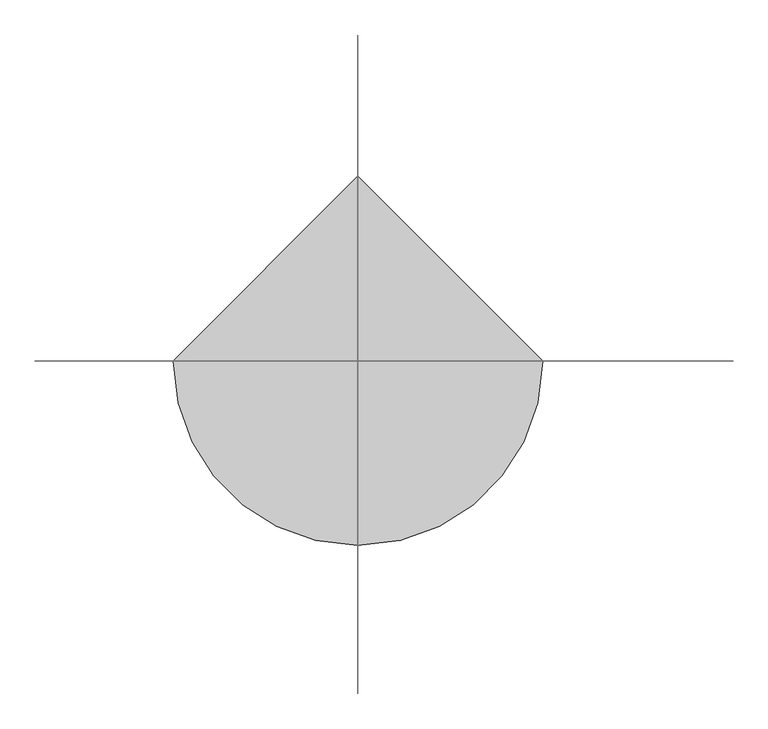
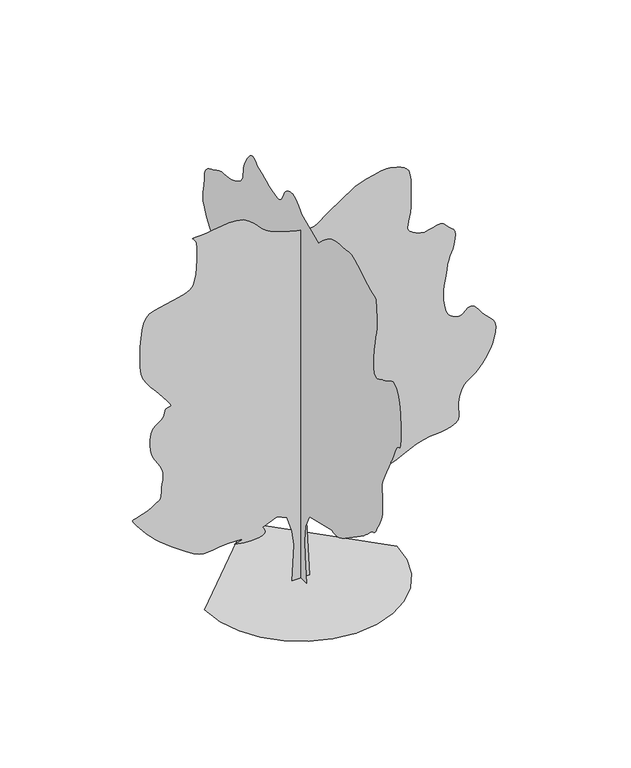
"""IFC4 building model written with IfcOpenShell, lengths in millimetres: geographic element geometry, RPC 木 - 落葉樹 : アメリカブナ - 6.0 メートル."""

from ifc_helpers import new_model, si_unit, origin, place, context, project, spatial, triangles, source, transform, mapped, element, save


def geographic_element_192016b0(model_context):
    return source(origin(), model_context, "Body", "Tessellation", [
        triangles([(0.0009733, 134.7013619, 0.0), (0.0009733, -147.494867, 0.0), (0.0009733, -109.8685844, 413.8878181), (0.0009733, -100.4623272, 649.050499), (0.0009733, -119.2748417, 884.2131798), (0.0009733, -232.153435, 1100.5633461), (0.0009733, -805.9506603, 1241.6609837), (0.0009733, -836.5581671, 1230.0334957), (0.0009733, -869.3831984, 1221.2035114), (0.0009733, -906.6532345, 1217.965991), (0.0009733, -950.5882708, 1223.1234524), (0.0009733, -1003.4058317, 1239.4685303), (0.0009733, -1067.3308542, 1269.7985104), (0.0009733, -1144.5859497, 1316.9135124), (0.0009733, -1455.0011593, 1533.2636787), (0.0009733, -1498.8811844, 1564.1163013), (0.0009733, -1542.2661816, 1593.486311), (0.0009733, -1585.8162849, 1623.3513485), (0.0009733, -1630.1888672, 1655.6862934), (0.0009733, -1676.041301, 1692.4613743), (0.0009733, -1724.0338657, 1735.6539413), (0.0009733, -1774.8239342, 1787.2388741), (0.0009733, -1818.8389801, 1828.7590141), (0.0009733, -1849.3615356, 1847.5739994), (0.0009733, -1871.3289448, 1854.3740204), (0.0009733, -1889.6765167, 1859.8590054), (0.0009733, -1909.3389793, 1874.723941), (0.0009733, -1935.2541126, 1909.6614887), (0.0009733, -1972.3591152, 1975.3715767), (0.0009733, -2012.7566494, 2050.40159), (0.0009733, -2045.5841515, 2111.4491718), (0.0009733, -2071.3341785, 2166.4067184), (0.0009733, -2090.5042294, 2223.1767998), (0.0009733, -2103.5867157, 2289.651812), (0.0009733, -2111.0717239, 2373.7344704), (0.0009733, -2113.4592236, 2483.3219673), (0.0009733, -2108.7967175, 2583.5521866), (0.0009733, -2099.1991928, 2645.9521568), (0.0009733, -2091.2441551, 2687.927211), (0.0009733, -2091.5191383, 2726.9521545), (0.0009733, -2106.6016479, 2780.4520866), (0.0009733, -2143.0767471, 2865.9023941), (0.0009733, -2207.5242668, 3000.6773071), (0.0009733, -2272.3543213, 3131.8524399), (0.0009733, -2311.5169018, 3208.0524399), (0.0009733, -2333.894315, 3249.2275429), (0.0009733, -2348.3743904, 3275.2526985), (0.0009733, -2363.8419056, 3306.0525627), (0.0009733, -2389.1819286, 3361.5276649), (0.0009733, -2433.2793823, 3461.6026611), (0.0009733, -2483.0818657, 3552.8029083), (0.0009733, -2520.7019531, 3587.7528099), (0.0009733, -2547.8020432, 3595.3779259), (0.0009733, -2566.002095, 3604.6529411), (0.0009733, -2576.9770065, 3644.5278328), (0.0009733, -2582.3519691, 3743.9528687), (0.0009733, -2583.7771729, 3931.9280228), (0.0009733, -2574.1771774, 4144.4034256), (0.0009733, -2548.4520035, 4302.6033623), (0.0009733, -2511.2269501, 4413.2285866), (0.0009733, -2467.0668549, 4483.053685), (0.0009733, -2420.6093708, 4518.8035378), (0.0009733, -2376.4568333, 4527.2536034), (0.0009733, -2339.2143391, 4515.1284714), (0.0009733, -2306.9368034, 4495.0285355), (0.0009733, -2274.4943069, 4475.2535797), (0.0009733, -2241.7217434, 4456.1535828), (0.0009733, -2208.456768, 4438.0035278), (0.0009733, -2174.5318039, 4421.2036812), (0.0009733, -2139.7866863, 4406.0284447), (0.0009733, -2104.0516582, 4392.8533768), (0.0009733, -2063.4090809, 4373.6783844), (0.0009733, -2017.3366024, 4348.9034431), (0.0009733, -1970.769096, 4331.3783501), (0.0009733, -1928.6465218, 4333.9284851), (0.0009733, -1895.9015728, 4369.4033546), (0.0009733, -1877.4714478, 4450.6036308), (0.0009733, -1878.294072, 4590.3785294), (0.0009733, -1893.3515831, 4743.5287743), (0.0009733, -1912.3565277, 4862.9287537), (0.0009733, -1932.3490574, 4958.6287262), (0.0009733, -1950.3665623, 5040.6789505), (0.0009733, -1963.4490486, 5119.1288132), (0.0009733, -1968.6315811, 5203.9794479), (0.0009733, -1962.9540207, 5305.2790787), (0.0009733, -1955.0840069, 5402.479541), (0.0009733, -1951.8190899, 5472.3543457), (0.0009733, -1947.4040977, 5521.0042831), (0.0009733, -1936.0790623, 5554.5045639), (0.0009733, -1912.0815445, 5578.9792328), (0.0009733, -1869.6565178, 5600.4796646), (0.0009733, -1803.044014, 5625.1043243), (0.0009733, -1720.9064404, 5661.3794357), (0.0009733, -1636.6338226, 5709.179425), (0.0009733, -1551.5337845, 5761.6047134), (0.0009733, -1466.931245, 5811.7045624), (0.0009733, -1384.1386242, 5852.579393), (0.0009733, -1304.4711033, 5877.3546249), (0.0009733, -1229.2460438, 5879.0795197), (0.0009733, -1155.7484224, 5869.4295273), (0.0009733, -1081.2633614, 5862.9049255), (0.0009733, -1007.1082947, 5856.8547134), (0.0009733, -934.5982584, 5848.679631), (0.0009733, -865.0506866, 5835.7548386), (0.0009733, -799.7806154, 5815.4049179), (0.0009733, -740.1056242, 5785.0044479), (0.0009733, -686.9580688, 5749.2798843), (0.0009733, -639.7330444, 5714.5296799), (0.0009733, -597.445473, 5680.604425), (0.0009733, -559.105444, 5647.3547104), (0.0009733, -523.727916, 5614.5793854), (0.0009733, -490.3253763, 5582.1296219), (0.0009733, -457.9103491, 5549.8542664), (0.0009733, -15.8033629, 5737.9794113), (0.0009733, 22.480868, 5779.9547562), (0.0009733, 60.6827967, 5819.9046432), (0.0009733, 98.7203278, 5855.7047836), (0.0009733, 136.5108627, 5885.354718), (0.0009733, 173.9723933, 5906.7795731), (0.0009733, 211.0226754, 5917.9044754), (0.0009733, 247.5792013, 5916.7045486), (0.0009733, 282.6827272, 5907.9045044), (0.0009733, 315.3177446, 5896.9545914), (0.0009733, 345.3202738, 5882.8798691), (0.0009733, 372.5252993, 5864.7048157), (0.0009733, 396.7678239, 5841.4294922), (0.0009733, 417.8828505, 5812.054541), (0.0009733, 435.7103597, 5775.6044403), (0.0009733, 452.7128466, 5735.1795822), (0.0009733, 472.6778707, 5696.4046234), (0.0009733, 497.4153869, 5662.079393), (0.0009733, 528.7329157, 5634.979303), (0.0009733, 568.4429555, 5617.9047638), (0.0009733, 618.3554976, 5613.7044388), (0.0009733, 680.2805695, 5625.1043243), (0.0009733, 747.7156248, 5646.6297546), (0.0009733, 813.1781261, 5670.6294525), (0.0009733, 876.993199, 5696.6796066), (0.0009733, 939.4932358, 5724.37966), (0.0009733, 1001.0058329, 5753.3046387), (0.0009733, 1061.8608393, 5783.054567), (0.0009733, 1122.385924, 5813.2294693), (0.0009733, 1150.6609423, 5838.9296448), (0.0009733, 1179.2634115, 5861.579425), (0.0009733, 1208.5259422, 5878.1545761), (0.0009733, 1238.7735146, 5885.5797043), (0.0009733, 1270.3410645, 5880.8299942), (0.0009733, 1303.5511013, 5860.8794678), (0.0009733, 1338.7360176, 5822.6294769), (0.0009733, 1373.2086227, 5775.8044281), (0.0009733, 1403.7311783, 5731.2548218), (0.0009733, 1429.8111271, 5687.8795624), (0.0009733, 1450.9562027, 5644.4793045), (0.0009733, 1466.6712318, 5599.9546967), (0.0009733, 1476.4611866, 5553.1046494), (0.0009733, 1479.8336552, 5502.8042313), (0.0009733, 1483.4812523, 5452.1044189), (0.0009733, 1495.191148, 5404.7044052), (0.0009733, 1516.1161789, 5360.4042023), (0.0009733, 1547.4087456, 5319.0793991), (0.0009733, 1590.2163071, 5280.554425), (0.0009733, 1645.6963509, 5244.6542908), (0.0009733, 1714.996336, 5211.204007), (0.0009733, 1788.9063595, 5186.2043701), (0.0009733, 1858.2064899, 5172.3790512), (0.0009733, 1924.0515987, 5164.8039322), (0.0009733, 1987.5940865, 5158.5543137), (0.0009733, 2049.9841736, 5148.679335), (0.0009733, 2112.3742607, 5130.2542969), (0.0009733, 2175.9167484, 5098.32892), (0.0009733, 2240.5017597, 5064.3292511), (0.0009733, 2303.2743816, 5038.2291), (0.0009733, 2361.2769459, 5012.9289001), (0.0009733, 2411.5469879, 4981.4040802), (0.0009733, 2451.1195724, 4936.5289124), (0.0009733, 2477.0345604, 4871.2538269), (0.0009733, 2486.331958, 4778.503965), (0.0009733, 2492.5844833, 4683.078685), (0.0009733, 2506.4019539, 4608.2036041), (0.0009733, 2520.4019714, 4544.5287117), (0.0009733, 2527.1521408, 4482.6537094), (0.0009733, 2519.2520416, 4413.2285866), (0.0009733, 2489.2945679, 4326.8283371), (0.0009733, 2429.8919437, 4214.1282394), (0.0009733, 2356.3968658, 4101.0031677), (0.0009733, 2289.9743214, 4014.028244), (0.0009733, 2231.9442879, 3944.8531059), (0.0009733, 2183.6218014, 3885.0279785), (0.0009733, 2146.3266941, 3826.2030807), (0.0009733, 2121.3692059, 3759.9780533), (0.0009733, 2110.0716396, 3677.9528275), (0.0009733, 2115.5842392, 3588.602758), (0.0009733, 2136.8916595, 3505.6778778), (0.0009733, 2169.0617889, 3428.6526375), (0.0009733, 2207.1542313, 3357.0776459), (0.0009733, 2246.2317879, 3290.4526428), (0.0009733, 2281.3643818, 3228.2526604), (0.0009733, 2307.6092915, 3170.0024368), (0.0009733, 2333.0293968, 3130.6025162), (0.0009733, 2364.704353, 3115.0525932), (0.0009733, 2396.2143482, 3108.0524391), (0.0009733, 2421.1443672, 3094.3024063), (0.0009733, 2433.074453, 3058.5275551), (0.0009733, 2425.586974, 2985.3773689), (0.0009733, 2392.2669147, 2859.5771988), (0.0009733, 2346.3593971, 2717.8521286), (0.0009733, 2303.741795, 2602.2772064), (0.0009733, 2261.946817, 2505.6519997), (0.0009733, 2218.506736, 2420.6843662), (0.0009733, 2170.9542606, 2340.1668972), (0.0009733, 2116.8167221, 2256.8517792), (0.0009733, 2053.6316254, 2163.5016632), (0.0009733, 1990.2540985, 2069.4091507), (0.0009733, 1937.0790012, 1987.8215435), (0.0009733, 1893.941518, 1917.4240963), (0.0009733, 1860.6739265, 1856.8965408), (0.0009733, 1837.1164982, 1804.928928), (0.0009733, 1823.1039814, 1760.1989548), (0.0009733, 1818.4689445, 1721.3939106), (0.0009733, 1822.4189941, 1694.76385), (0.0009733, 1831.633984, 1682.286414), (0.0009733, 1842.1640099, 1676.2263187), (0.0009733, 1850.0614929, 1668.8488621), (0.0009733, 1851.3789997, 1652.4213764), (0.0009733, 1842.1640099, 1619.2113396), (0.0009733, 1818.4689445, 1561.4837585), (0.0009733, 1798.7513981, 1500.5736683), (0.0009733, 1796.6388817, 1458.9161819), (0.0009733, 1800.9439968, 1430.4235897), (0.0009733, 1800.4789089, 1409.0036762), (0.0009733, 1784.0514233, 1388.5736732), (0.0009733, 1740.4738506, 1363.0410748), (0.0009733, 1658.5587925, 1326.3210777), (0.0009733, 1569.2912762, 1288.8036003), (0.0009733, 1504.2137077, 1262.3110313), (0.0009733, 1452.9586967, 1242.8959373), (0.0009733, 1405.1585621, 1226.6059433), (0.0009733, 1350.4460587, 1209.4934704), (0.0009733, 1278.4585922, 1187.608469), (0.0009733, 1178.8259382, 1157.003433), (0.0009733, 1078.8083513, 1127.6584219), (0.0009733, 1006.4358067, 1109.9959099), (0.0009733, 952.4932417, 1100.7283796), (0.0009733, 907.7631958, 1096.558358), (0.0009733, 863.0356934, 1094.2008711), (0.0009733, 809.0906576, 1090.3608438), (0.0009733, 736.7181129, 1081.7508316), (0.0009733, 652.0604897, 1068.0108273), (0.0009733, 567.4004683, 1051.3083584), (0.0009733, 482.7428813, 1032.140851), (0.0009733, 398.0828236, 1010.9957754), (0.0009733, 313.4252366, 988.3707756), (0.0009733, 228.7664324, 964.7582634), (0.0009733, 144.1076192, 940.6532667), (134.0396109, 0.0003104, 0.0138465), (-129.3426047, 0.0003104, 0.0138465), (-101.123079, 0.0002775, 554.9979549), (-129.3426047, 0.000265, 780.7556139), (-204.5949064, 0.0002508, 1015.9182947), (-355.1002728, 0.0002461, 1091.1708961), (-571.4504391, 0.0002508, 997.1057802), (-553.8429382, 0.0002524, 972.9983128), (-539.4454159, 0.000254, 949.3882713), (-531.465416, 0.0002555, 926.7632715), (-533.1104101, 0.0002571, 905.6181959), (-547.5904492, 0.0002587, 886.4482178), (-578.1129684, 0.0002587, 869.7482197), (-627.8879826, 0.0002602, 856.0082153), (-686.4380424, 0.0002602, 846.9306444), (-741.5356241, 0.0002602, 843.2831926), (-793.7506056, 0.0002602, 844.1606827), (-843.663184, 0.0002602, 848.6581553), (-891.8481789, 0.0002602, 855.8706511), (-938.8807732, 0.0002587, 864.8932108), (-985.3357864, 0.0002587, 874.8207298), (-938.2757229, 0.0002587, 886.8056814), (-899.1156858, 0.0002571, 898.1307169), (-875.7482168, 0.0002571, 908.1407164), (-876.0782112, 0.0002555, 916.1757637), (-908.000754, 0.0002555, 921.5782682), (-979.4132555, 0.0002555, 923.690712), (-1098.2133442, 0.0002555, 921.8532515), (-1223.378524, 0.0002571, 913.2156973), (-1316.2934921, 0.0002571, 899.9682501), (-1388.4736794, 0.0002571, 889.0256767), (-1451.4387314, 0.0002571, 887.2982386), (-1516.7087299, 0.0002571, 901.6956882), (-1595.8012859, 0.0002555, 939.1307579), (-1700.2313942, 0.0002508, 1006.5108021), (-1816.016478, 0.0002461, 1088.4284037), (-1921.6016029, 0.0002414, 1165.4084433), (-2017.1466431, 0.0002367, 1238.2735451), (-2102.8191753, 0.0002336, 1307.8509842), (-2178.7867767, 0.0002289, 1374.9560452), (-2245.2068504, 0.0002242, 1440.4186192), (-2302.2492989, 0.0002211, 1505.0587143), (-2354.1368294, 0.0002179, 1567.5838223), (-2402.8969345, 0.0002132, 1625.1762371), (-2445.4045143, 0.0002101, 1676.3488403), (-2478.5318527, 0.0002085, 1719.6238152), (-2499.1544312, 0.0002069, 1753.5214554), (-2504.1520912, 0.0002054, 1776.5588573), (-2490.3793854, 0.0002038, 1787.2539894), (-2459.3920326, 0.0002038, 1794.0263958), (-2417.5419708, 0.0002038, 1805.7364368), (-2368.9443558, 0.0002022, 1821.5614883), (-2317.716814, 0.0002007, 1840.6764553), (-2267.9692692, 0.0001991, 1862.2590042), (-2223.8167316, 0.0001991, 1885.4865108), (-2189.3717411, 0.0001975, 1909.5389671), (-2162.3867603, 0.000196, 1927.8015152), (-2138.1966671, 0.000196, 1938.169051), (-2117.2992508, 0.0001944, 1946.561562), (-2100.1866325, 0.0001944, 1958.9015064), (-2087.3541309, 0.0001928, 1981.1165749), (-2079.291687, 0.0001897, 2019.1266094), (-2076.4941833, 0.0001866, 2078.8566845), (-2072.5992176, 0.0001834, 2146.7042873), (-2063.769088, 0.0001787, 2206.9817127), (-2054.2791149, 0.0001756, 2262.4893711), (-2048.4115952, 0.0001725, 2316.0218594), (-2050.4417038, 0.0001693, 2370.3768265), (-2064.6466507, 0.0001662, 2428.3494507), (-2095.3066978, 0.0001615, 2492.7420319), (-2134.2492336, 0.0001583, 2555.8271347), (-2169.5717869, 0.0001552, 2611.5022247), (-2199.9567055, 0.0001521, 2665.0271553), (-2224.0917149, 0.0001489, 2721.6771858), (-2240.6542213, 0.0001442, 2786.727285), (-2248.3342758, 0.0001395, 2865.4274231), (-2245.8117554, 0.0001348, 2963.0772766), (-2228.8892418, 0.0001286, 3053.9275452), (-2197.981826, 0.0001254, 3115.1525871), (-2158.6842247, 0.0001223, 3156.3273994), (-2116.5866489, 0.0001207, 3186.952565), (-2077.289193, 0.0001191, 3216.6024994), (-2046.3816319, 0.000116, 3254.8024933), (-2029.4615891, 0.0001129, 3311.1025452), (-2011.7716805, 0.0001113, 3359.2778023), (-1982.4015255, 0.0001097, 3377.3025742), (-1952.6991234, 0.0001097, 3381.2026268), (-1934.0241005, 0.0001082, 3386.9025696), (-1937.7264908, 0.0001082, 3410.3775902), (-1975.1615604, 0.0001035, 3467.6028763), (-2057.6791981, 9.72e-05, 3574.5027466), (-2156.9017754, 9.09e-05, 3694.6029739), (-2237.5292667, 8.47e-05, 3789.0530228), (-2300.5494026, 8e-05, 3870.1780128), (-2346.9519482, 7.53e-05, 3950.303064), (-2377.7218723, 7.05e-05, 4041.8032928), (-2393.8469055, 6.27e-05, 4156.9782394), (-2396.3144875, 5.33e-05, 4308.2033112), (-2391.2694466, 4.39e-05, 4470.0786049), (-2382.4394623, 3.61e-05, 4609.2538307), (-2367.1893757, 2.98e-05, 4726.0536781), (-2342.8918762, 2.35e-05, 4820.8039993), (-2306.911805, 1.88e-05, 4893.8541916), (-2256.6142937, 1.57e-05, 4945.4789474), (-2189.3717411, 1.41e-05, 4976.0538254), (-2104.7391163, 1.25e-05, 4994.8788391), (-2008.7541321, 1.25e-05, 5012.5289246), (-1908.491502, 1.1e-05, 5031.3539383), (-1811.0265209, 9.4e-06, 5053.6293228), (-1723.4339024, 7.8e-06, 5081.653775), (-1652.7887959, 6.3e-06, 5117.7288986), (-1606.1663509, 3.1e-06, 5164.2039688), (-1578.8513031, -1.6e-06, 5232.7044388), (-1560.4237942, -6.3e-06, 5326.3795349), (-1549.3987404, -1.25e-05, 5434.7043182), (-1544.298761, -2.04e-05, 5547.1544312), (-1543.6387722, -2.67e-05, 5653.1793549), (-1545.9437187, -3.14e-05, 5742.2547318), (-1549.7288074, -3.45e-05, 5803.8294617), (-1560.9438206, -3.76e-05, 5842.6794159), (-1580.7187763, -3.92e-05, 5871.4799835), (-1600.3263004, -4.08e-05, 5891.7049118), (-1611.0487564, -4.08e-05, 5904.879689), (-1604.1663277, -4.23e-05, 5912.4298096), (-1570.95382, -4.23e-05, 5915.9045975), (-1502.6962132, -4.23e-05, 5916.7295471), (-1406.2711395, -4.23e-05, 5923.0547424), (-1298.001004, -4.39e-05, 5937.4550262), (-1183.3109116, -4.39e-05, 5953.0046585), (-1067.6358501, -4.39e-05, 5962.7796432), (-956.4032501, -4.39e-05, 5959.9048187), (-855.043158, -4.39e-05, 5937.4550262), (-768.9856201, -4.08e-05, 5888.5045258), (-703.6355392, -3.61e-05, 5829.3546478), (-655.0655388, -3.29e-05, 5779.2298004), (-614.7254866, -3.14e-05, 5735.7045502), (-574.0554763, -2.82e-05, 5696.3046295), (-524.5004342, -2.67e-05, 5658.5546082), (-457.5028522, -2.35e-05, 5619.9546387), (-364.5052946, -2.19e-05, 5578.0792877), (-256.7552037, -1.88e-05, 5538.7543625), (-153.2841212, -1.72e-05, 5508.8044464), (-57.2167973, -1.57e-05, 5487.254599), (28.3195219, -1.57e-05, 5473.1042999), (100.1988258, -1.57e-05, 5465.3791901), (155.2941184, -1.41e-05, 5463.054332), (190.4793981, -1.57e-05, 5465.2042007), (215.8194211, -1.57e-05, 5473.054303), (243.4629373, -1.57e-05, 5487.6295761), (273.410219, -1.72e-05, 5507.6545166), (305.6602309, -1.88e-05, 5531.7792068), (340.2152802, -2.04e-05, 5558.729306), (377.0728051, -2.19e-05, 5587.1293167), (416.2353493, -2.35e-05, 5615.7043167), (792.4981384, -3.92e-05, 5869.679512), (817.2881224, -3.92e-05, 5878.9295288), (882.5581936, -4.08e-05, 5902.1548553), (974.6482847, -4.23e-05, 5932.6297394), (1079.9033426, -4.55e-05, 5963.5795944), (1184.6634453, -4.55e-05, 5988.3048294), (1275.2734669, -4.7e-05, 6000.0046967), (1338.0760288, -4.7e-05, 5991.9796051), (1385.3260517, -4.55e-05, 5975.0550568), (1436.1986732, -4.39e-05, 5961.4297256), (1487.4012165, -4.39e-05, 5946.3044861), (1535.6386791, -4.23e-05, 5924.9546265), (1577.6262325, -4.08e-05, 5892.5548599), (1610.068729, -3.76e-05, 5844.3798935), (1629.6788692, -3.29e-05, 5775.6294388), (1639.0838184, -2.82e-05, 5698.6044891), (1643.8838161, -2.51e-05, 5627.2047775), (1645.2263214, -2.04e-05, 5558.9042953), (1644.2663509, -1.72e-05, 5491.2793533), (1642.1538345, -1.25e-05, 5421.8545212), (1640.0437889, -7.8e-06, 5348.1293701), (1639.0838184, -3.1e-06, 5267.6790482), (1634.0912453, 1.6e-06, 5187.5792862), (1622.1912449, 6.3e-06, 5116.5539703), (1607.9838272, 9.4e-06, 5054.4042755), (1596.0812107, 1.25e-05, 5001.0040466), (1591.0912537, 1.57e-05, 4956.1288788), (1597.6187622, 1.72e-05, 4919.6537796), (1620.2713039, 1.88e-05, 4891.4037598), (1651.9738747, 2.04e-05, 4868.9289688), (1682.6888603, 2.19e-05, 4849.728978), (1712.5813671, 2.19e-05, 4833.6537964), (1741.8138851, 2.35e-05, 4820.5537239), (1770.5564621, 2.35e-05, 4810.2287727), (1798.9665012, 2.51e-05, 4802.5539505), (1827.213905, 2.51e-05, 4797.3289787), (1863.2490601, 2.51e-05, 4800.3037971), (1911.6264851, 2.35e-05, 4812.9788956), (1967.4065105, 2.35e-05, 4828.9287941), (2025.6565887, 2.19e-05, 4841.7788818), (2081.4366142, 2.19e-05, 4845.0539726), (2129.8141846, 2.35e-05, 4832.3788742), (2165.8491943, 2.51e-05, 4797.3289787), (2195.3593117, 2.67e-05, 4758.0787582), (2225.6892918, 2.82e-05, 4731.9538994), (2254.2093533, 2.98e-05, 4711.4536972), (2278.2892788, 3.14e-05, 4688.9536171), (2295.2918747, 3.29e-05, 4656.9288277), (2302.5867783, 3.61e-05, 4607.7786301), (2297.5418827, 4.08e-05, 4533.9534851), (2283.3617889, 4.55e-05, 4455.6536133), (2265.8942505, 4.86e-05, 4393.6536186), (2246.4493618, 5.17e-05, 4341.2033318), (2226.3468098, 5.49e-05, 4291.5284569), (2206.9042465, 5.8e-05, 4237.9035324), (2189.4342373, 6.27e-05, 4173.6033875), (2175.2567596, 6.74e-05, 4091.8531448), (2162.3117649, 7.21e-05, 4004.3782516), (2148.874213, 7.68e-05, 3925.278138), (2136.7516972, 8.15e-05, 3851.452993), (2127.756752, 8.62e-05, 3779.753009), (2123.6991508, 8.94e-05, 3707.0780846), (2126.3866322, 9.41e-05, 3630.302829), (2137.6292599, 9.88e-05, 3546.2777252), (2155.4842747, 0.0001035, 3469.5027603), (2176.791695, 0.0001066, 3413.652681), (2201.5542824, 0.0001097, 3374.2527603), (2229.7742168, 0.0001113, 3346.8526886), (2261.4493183, 0.0001129, 3327.0277359), (2296.5817669, 0.0001129, 3310.302594), (2335.1669117, 0.0001144, 3292.3025299), (2374.57439, 0.0001144, 3289.8526794), (2413.1618603, 0.0001129, 3313.0777153), (2452.4043777, 0.0001113, 3347.3276596), (2493.7893517, 0.0001097, 3377.9778236), (2538.8020111, 0.0001082, 3390.3276512), (2588.9021507, 0.0001097, 3369.8027412), (2645.5771797, 0.0001144, 3301.7025375), (2706.5522369, 0.0001191, 3218.4776756), (2765.8771042, 0.0001223, 3156.4523918), (2819.5773148, 0.0001254, 3106.9525063), (2863.7772331, 0.0001286, 3061.2523888), (2894.4523956, 0.0001317, 3010.6022827), (2907.702459, 0.0001348, 2946.27743), (2899.552375, 0.0001411, 2859.6021973), (2878.1022308, 0.0001458, 2766.3520752), (2853.5522758, 0.0001505, 2686.1020317), (2825.0272728, 0.0001552, 2615.7519653), (2791.7272705, 0.0001583, 2552.1270699), (2752.8273193, 0.0001615, 2492.1121284), (2707.5271774, 0.0001662, 2432.6019527), (2654.9771873, 0.0001693, 2370.4569088), (2600.8270042, 0.0001725, 2317.1443199), (2551.1021324, 0.0001756, 2280.2868313), (2505.6519997, 0.0001772, 2250.9967587), (2464.3344635, 0.0001787, 2220.3917953), (2426.9544777, 0.0001803, 2179.5842571), (2393.3594353, 0.000185, 2119.691692), (2363.3868462, 0.0001897, 2031.8240902), (2347.2343437, 0.000196, 1934.7965824), (2348.1943142, 0.0002007, 1852.2490047), (2355.7344063, 0.0002038, 1782.5363995), (2359.3269196, 0.0002085, 1724.0138088), (2348.4393574, 0.0002116, 1675.0338043), (2312.5418392, 0.0002132, 1633.9512829), (2241.1017231, 0.0002148, 1599.1237576), (2155.26423, 0.0002164, 1575.9487186), (2078.4766205, 0.0002179, 1565.7737583), (2003.661565, 0.0002179, 1560.866209), (1923.7465302, 0.0002179, 1553.4887524), (1831.6565117, 0.0002195, 1535.9111916), (1720.3138893, 0.0002211, 1500.3962082), (1582.6438042, 0.0002258, 1439.2111347), (1432.7436516, 0.0002289, 1368.8411568), (1291.0710491, 0.000232, 1310.483527), (1160.0909626, 0.0002352, 1263.4785473), (1042.2783136, 0.0002383, 1227.1685543), (940.0957426, 0.0002399, 1200.8959574), (856.0131569, 0.0002399, 1184.000913), (792.4981384, 0.0002414, 1175.8284468), (397.4228348, 0.0002414, 1166.4234249), (105.8200852, 0.0002446, 1119.3909033), (87.0075707, 0.0002587, 865.4131645), (-1430.8636791, 0.0, 0.0118397), (-1393.0360462, -327.8602567, 0.0118397), (-1285.305994, -628.9454762, 0.0118397), (-1116.2958887, -894.6331833, 0.0118397), (-894.6331833, -1116.2958887, 0.0118397), (-628.9454762, -1285.305994, 0.0118397), (-327.8602567, -1393.0360462, 0.0118397), (6.25e-05, -1430.8636791, 0.0118397), (327.8602567, -1393.0360462, 0.0118397), (628.9454762, -1285.305994, 0.0118397), (894.6331833, -1116.2958887, 0.0118397), (1116.2958887, -894.6331833, 0.0118397), (1285.305994, -628.9454762, 0.0118397), (1393.0360462, -327.8602567, 0.0118397), (1430.8636791, 0.0001254, 0.0118397), (-0.0001876, 1430.8636791, 0.0118397)], [[1, 2, 3], [254, 1, 3], [254, 3, 4], [254, 4, 5], [254, 5, 6], [53, 54, 55], [52, 53, 55], [201, 202, 203], [201, 203, 204], [200, 201, 204], [222, 223, 224], [52, 55, 56], [200, 204, 205], [199, 200, 205], [253, 254, 6], [221, 222, 224], [221, 224, 225], [229, 230, 231], [229, 231, 232], [228, 229, 232], [228, 232, 233], [227, 228, 233], [252, 253, 6], [221, 225, 226], [220, 221, 226], [199, 205, 206], [198, 199, 206], [62, 63, 64], [61, 62, 64], [61, 64, 65], [60, 61, 65], [60, 65, 66], [59, 60, 66], [59, 66, 67], [59, 67, 68], [58, 59, 68], [58, 68, 69], [58, 69, 70], [57, 58, 70], [57, 70, 71], [57, 71, 72], [57, 72, 73], [57, 73, 74], [56, 57, 74], [52, 56, 74], [51, 52, 74], [50, 51, 74], [50, 74, 75], [49, 50, 75], [48, 49, 75], [47, 48, 75], [46, 47, 75], [45, 46, 75], [44, 45, 75], [43, 44, 75], [42, 43, 75], [42, 75, 76], [41, 42, 76], [227, 233, 234], [226, 227, 234], [220, 226, 234], [219, 220, 234], [219, 234, 235], [219, 235, 236], [219, 236, 237], [218, 219, 237], [218, 237, 238], [218, 238, 239], [218, 239, 240], [217, 218, 240], [217, 240, 241], [217, 241, 242], [217, 242, 243], [217, 243, 244], [217, 244, 245], [217, 245, 246], [216, 217, 246], [216, 246, 247], [215, 216, 247], [215, 247, 248], [251, 252, 6], [88, 89, 90], [88, 90, 91], [87, 88, 91], [87, 91, 92], [86, 87, 92], [86, 92, 93], [85, 86, 93], [84, 85, 93], [84, 93, 94], [83, 84, 94], [82, 83, 94], [81, 82, 94], [81, 94, 95], [80, 81, 95], [80, 95, 96], [80, 96, 97], [80, 97, 98], [80, 98, 99], [80, 99, 100], [80, 100, 101], [80, 101, 102], [80, 102, 103], [80, 103, 104], [80, 104, 105], [80, 105, 106], [80, 106, 107], [80, 107, 108], [80, 108, 109], [80, 109, 110], [80, 110, 111], [80, 111, 112], [79, 80, 112], [79, 112, 113], [78, 79, 113], [77, 78, 113], [76, 77, 113], [41, 76, 113], [40, 41, 113], [40, 113, 114], [39, 40, 114], [198, 206, 207], [197, 198, 207], [196, 197, 207], [196, 207, 208], [195, 196, 208], [195, 208, 209], [195, 209, 210], [195, 210, 211], [194, 195, 211], [194, 211, 212], [194, 212, 213], [193, 194, 213], [193, 213, 214], [214, 215, 248], [193, 214, 248], [193, 248, 249], [192, 193, 249], [192, 249, 250], [192, 250, 251], [192, 251, 6], [192, 6, 7], [191, 192, 7], [190, 191, 7], [189, 190, 7], [38, 39, 114], [37, 38, 114], [36, 37, 114], [35, 36, 114], [34, 35, 114], [33, 34, 114], [32, 33, 114], [31, 32, 114], [30, 31, 114], [29, 30, 114], [28, 29, 114], [27, 28, 114], [26, 27, 114], [25, 26, 114], [24, 25, 114], [23, 24, 114], [22, 23, 114], [21, 22, 114], [20, 21, 114], [19, 20, 114], [18, 19, 114], [17, 18, 114], [16, 17, 114], [15, 16, 114], [14, 15, 114], [13, 14, 114], [12, 13, 114], [11, 12, 114], [10, 11, 114], [9, 10, 114], [8, 9, 114], [7, 8, 114], [189, 7, 114], [188, 189, 114], [188, 114, 115], [188, 115, 116], [188, 116, 117], [188, 117, 118], [188, 118, 119], [188, 119, 120], [188, 120, 121], [146, 147, 148], [145, 146, 148], [144, 145, 148], [144, 148, 149], [143, 144, 149], [143, 149, 150], [142, 143, 150], [142, 150, 151], [142, 151, 152], [141, 142, 152], [141, 152, 153], [141, 153, 154], [141, 154, 155], [141, 155, 156], [140, 141, 156], [140, 156, 157], [139, 140, 157], [138, 139, 157], [138, 157, 158], [137, 138, 158], [137, 158, 159], [136, 137, 159], [135, 136, 159], [135, 159, 160], [134, 135, 160], [134, 160, 161], [174, 175, 176], [173, 174, 176], [173, 176, 177], [172, 173, 177], [171, 172, 177], [171, 177, 178], [170, 171, 178], [170, 178, 179], [169, 170, 179], [168, 169, 179], [167, 168, 179], [166, 167, 179], [165, 166, 179], [165, 179, 180], [165, 180, 181], [165, 181, 182], [165, 182, 183], [165, 183, 184], [165, 184, 185], [165, 185, 186], [165, 186, 187], [164, 165, 187], [164, 187, 188], [163, 164, 188], [162, 163, 188], [161, 162, 188], [134, 161, 188], [133, 134, 188], [132, 133, 188], [125, 126, 127], [124, 125, 127], [124, 127, 128], [123, 124, 128], [122, 123, 128], [121, 122, 128], [121, 128, 129], [121, 129, 130], [121, 130, 131], [188, 121, 131], [132, 188, 131], [274, 275, 276], [531, 255, 256], [531, 256, 257], [531, 257, 258], [531, 258, 259], [530, 531, 259], [376, 377, 378], [376, 378, 379], [375, 376, 379], [273, 274, 276], [273, 276, 277], [375, 379, 380], [374, 375, 380], [273, 277, 278], [272, 273, 278], [301, 302, 303], [301, 303, 304], [300, 301, 304], [300, 304, 305], [299, 300, 305], [299, 305, 306], [298, 299, 306], [298, 306, 307], [297, 298, 307], [297, 307, 308], [271, 272, 278], [296, 297, 308], [296, 308, 309], [373, 374, 380], [373, 380, 381], [372, 373, 381], [295, 296, 309], [295, 309, 310], [294, 295, 310], [294, 310, 311], [294, 311, 312], [294, 312, 313], [293, 294, 313], [293, 313, 314], [292, 293, 314], [271, 278, 279], [291, 292, 314], [530, 259, 260], [372, 381, 382], [371, 372, 382], [291, 314, 315], [290, 291, 315], [371, 382, 383], [370, 371, 383], [370, 383, 384], [369, 370, 384], [369, 384, 385], [369, 385, 386], [369, 386, 387], [369, 387, 388], [369, 388, 389], [369, 389, 390], [368, 369, 390], [368, 390, 391], [367, 368, 391], [367, 391, 392], [367, 392, 393], [366, 367, 393], [366, 393, 394], [270, 271, 279], [366, 394, 395], [338, 339, 340], [338, 340, 341], [289, 290, 315], [483, 484, 485], [483, 485, 486], [482, 483, 486], [481, 482, 486], [481, 486, 487], [480, 481, 487], [288, 289, 315], [287, 288, 315], [286, 287, 315], [285, 286, 315], [284, 285, 315], [283, 284, 315], [282, 283, 315], [282, 315, 316], [281, 282, 316], [281, 316, 317], [281, 317, 318], [281, 318, 319], [281, 319, 320], [280, 281, 320], [280, 320, 321], [279, 280, 321], [279, 321, 322], [480, 487, 488], [264, 265, 266], [263, 264, 266], [263, 266, 267], [262, 263, 267], [262, 267, 268], [261, 262, 268], [261, 268, 269], [261, 269, 270], [261, 270, 279], [261, 279, 322], [260, 261, 322], [530, 260, 322], [530, 322, 323], [529, 530, 323], [529, 323, 324], [366, 395, 396], [365, 366, 396], [337, 338, 341], [337, 341, 342], [529, 324, 325], [528, 529, 325], [527, 528, 325], [526, 527, 325], [525, 526, 325], [524, 525, 325], [523, 524, 325], [522, 523, 325], [521, 522, 325], [521, 325, 326], [521, 326, 327], [521, 327, 328], [521, 328, 329], [521, 329, 330], [521, 330, 331], [521, 331, 332], [521, 332, 333], [521, 333, 334], [521, 334, 335], [521, 335, 336], [521, 336, 337], [521, 337, 342], [520, 521, 342], [520, 342, 343], [519, 520, 343], [518, 519, 343], [518, 343, 344], [517, 518, 344], [449, 450, 451], [448, 449, 451], [448, 451, 452], [447, 448, 452], [446, 447, 452], [446, 452, 453], [516, 517, 344], [515, 516, 344], [514, 515, 344], [513, 514, 344], [512, 513, 344], [511, 512, 344], [510, 511, 344], [509, 510, 344], [508, 509, 344], [507, 508, 344], [506, 507, 344], [505, 506, 344], [504, 505, 344], [503, 504, 344], [502, 503, 344], [501, 502, 344], [500, 501, 344], [499, 500, 344], [498, 499, 344], [497, 498, 344], [496, 497, 344], [495, 496, 344], [494, 495, 344], [493, 494, 344], [492, 493, 344], [491, 492, 344], [490, 491, 344], [489, 490, 344], [488, 489, 344], [480, 488, 344], [479, 480, 344], [478, 479, 344], [477, 478, 344], [476, 477, 344], [475, 476, 344], [474, 475, 344], [473, 474, 344], [472, 473, 344], [471, 472, 344], [470, 471, 344], [469, 470, 344], [468, 469, 344], [467, 468, 344], [466, 467, 344], [465, 466, 344], [464, 465, 344], [463, 464, 344], [463, 344, 345], [462, 463, 345], [462, 345, 346], [461, 462, 346], [460, 461, 346], [459, 460, 346], [458, 459, 346], [457, 458, 346], [456, 457, 346], [455, 456, 346], [454, 455, 346], [453, 454, 346], [446, 453, 346], [445, 446, 346], [444, 445, 346], [443, 444, 346], [442, 443, 346], [441, 442, 346], [440, 441, 346], [439, 440, 346], [438, 439, 346], [437, 438, 346], [436, 437, 346], [435, 436, 346], [435, 346, 347], [435, 347, 348], [435, 348, 349], [435, 349, 350], [435, 350, 351], [435, 351, 352], [435, 352, 353], [435, 353, 354], [435, 354, 355], [435, 355, 356], [435, 356, 357], [435, 357, 358], [435, 358, 359], [435, 359, 360], [435, 360, 361], [435, 361, 362], [435, 362, 363], [435, 363, 364], [435, 364, 365], [435, 365, 396], [435, 396, 397], [435, 397, 398], [435, 398, 399], [435, 399, 400], [435, 400, 401], [435, 401, 402], [435, 402, 403], [435, 403, 404], [435, 404, 405], [435, 405, 406], [435, 406, 407], [435, 407, 408], [435, 408, 409], [434, 435, 409], [433, 434, 409], [432, 433, 409], [431, 432, 409], [430, 431, 409], [429, 430, 409], [429, 409, 410], [429, 410, 411], [429, 411, 412], [428, 429, 412], [428, 412, 413], [427, 428, 413], [426, 427, 413], [426, 413, 414], [425, 426, 414], [425, 414, 415], [425, 415, 416], [425, 416, 417], [424, 425, 417], [424, 417, 418], [423, 424, 418], [423, 418, 419], [422, 423, 419], [422, 419, 420], [421, 422, 420], [546, 547, 532], [545, 546, 532], [545, 532, 533], [544, 545, 533], [544, 533, 534], [544, 534, 535], [543, 544, 535], [542, 543, 535], [542, 535, 536], [542, 536, 537], [542, 537, 538], [542, 538, 539], [542, 539, 540], [542, 540, 541]], closed=False),
    ])


if __name__ == "__main__":
    model = new_model("IFC4")
    model_context = context("Model", 3, world=origin())
    ifc_project = project(units=[si_unit("LENGTHUNIT", "METRE", prefix="MILLI")], contexts=[model_context])
    site = spatial("IfcSite", under=ifc_project)
    building = spatial("IfcBuilding", under=site)
    placement = place(None, origin())
    geographic_element_shape = geographic_element_192016b0(model_context)
    element("IfcGeographicElement", 1, ObjectType="RPC 木 - 落葉樹 : アメリカブナ - 6.0 メートル", at=placement, inside=building, context=model_context, shape_type="MappedRepresentation", body=[
        mapped(geographic_element_shape, transform((0.0, 0.0, 0.0), x_axis=(1.0, 0.0, 0.0), y_axis=(0.0, 1.0, 0.0), z_axis=(0.0, 0.0, 1.0))),
    ])
    save(model, "model.ifc")

# Revit data of these elements
# Type "RPC 木 - 落葉樹 : アメリカブナ - 6.0 メートル"
#   built-in parameter 1005198 = "{2, 15},{39, RPC-16-G1GQ-43Q0-7NP3-0000-ST1L-LVER-AU},{1, 0},{1, 0},{2, 35},{1, 8},{5, Color},{1, 0},{1, 0},{3, 0.8},{3, 0.8},{3, 0.8},{1, 8},{7, BBoxMin},{1, 0},{1, 0},{1, 0},{1, 0},{1, 0},{1, 8},{7, BBoxMax},{1, 0},{1, 0},{1, 0},{1, 0},{1, 0},{2, 11},{9, RPCTypeId},{1, 0},{1, 0},{39, RPC-16-G1GQ-43Q0-7NP3-0000-ST1L-LVER-AU},{1, 6},{14, RPCPlantHeight},{1, 0},{1, 0},{6, 19.685},{2, 11},{7, keyword},{1, 0},{1, 0},{126, :Geometry:RPC:American Beech:Fagus grandifolia:The beech genus comprises about 10 species; American beech is native to Canada.},{2, 11},{8, category},{1, 0},{1, 0},{16, :Trees [General]},{2, 11},{12, LocalizedUID},{1, 0},{1, 0},{14, American Beech},{2, 14},{6, Height},{1, 0},{1, 0},{6, 19.685},{1, 2},{16, Cast Reflections},{1, 0},{1, 0},{1, 0},{1, 2},{12, Cast Shadows},{1, 0},{1, 0},{1, 1},{1, 2},{9, Lock View},{1, 0},{1, 0},{1, 0},{1, 4},{5, ViewC},{1, 0},{1, 0},{1, 0},{2, 11},{20, AdvancedUIDefinition},{1, 0},{1, 0},{0, },{2, 11},{10, AssetLibID},{1, 0},{1, 0},{36, 4D3F6E72-3F99-4203-98E9-AF80B3C7A7A4},{2, 11},{10, BaseSchema},{1, 0},{1, 0},{9, RPCSchema},{2, 11},{12, ExchangeGUID},{1, 0},{1, 0},{0, },{1, 2},{6, Hidden},{1, 0},{1, 0},{1, 0},{1, 4},{11, RPCCategory},{1, 0},{1, 0},{1, 0},{2, 11},{8, RPCImage},{1, 0},{1, 0},{0, },{1, 4},{13, SchemaVersion},{1, 0},{1, 0},{1, 4},{2, 11},{12, UIDefinition},{1, 0},{1, 0},{0, },{2, 11},{6, UIName},{1, 0},{1, 0},{39, RPC-16-G1GQ-43Q0-7NP3-0000-ST1L-LVER-AU},{2, 11},{11, VersionGUID},{1, 0},{1, 0},{9, RPCSchema},{2, 11},{9, assettype},{1, 0},{1, 0},{11, RPCGeometry},{2, 11},{11, description},{1, 0},{1, 0},{0, },{2, 11},{9, localname},{1, 0},{1, 0},{3, RPC},{2, 11},{9, localtype},{1, 0},{1, 0},{3, RPC},{1, 4},{8, revision},{1, 0},{1, 0},{1, 1},{2, 11},{9, thumbnail},{1, 0},{1, 0},{0, },{1, 4},{7, version},{1, 0},{1, 0},{1, 1},{1, 2},{20, RPC_Cast Reflections},{1, 0},{1, 0},{1, 1},{1, 2},{16, RPC_Cast Shadows},{1, 0},{1, 0},{1, 1},{1, 2},{13, RPC_Lock View},{1, 0},{1, 0},{1, 0},{1, 4},{9, RPC_ViewC},{1, 0},{1, 0},{1, 0},{21, assetlibrary_base.fbx},{1, 5},"
#   built-in parameter 1005195 = "RPC-16-G1GQ-43Q0-7NP3-0000-ST1L-LVER-AU"
#   Type Comments = "アメリカブナ"
#   Height = 6000 mm
#   Default Elevation = 0
